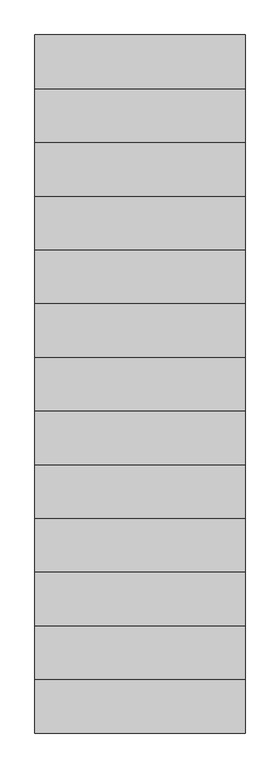
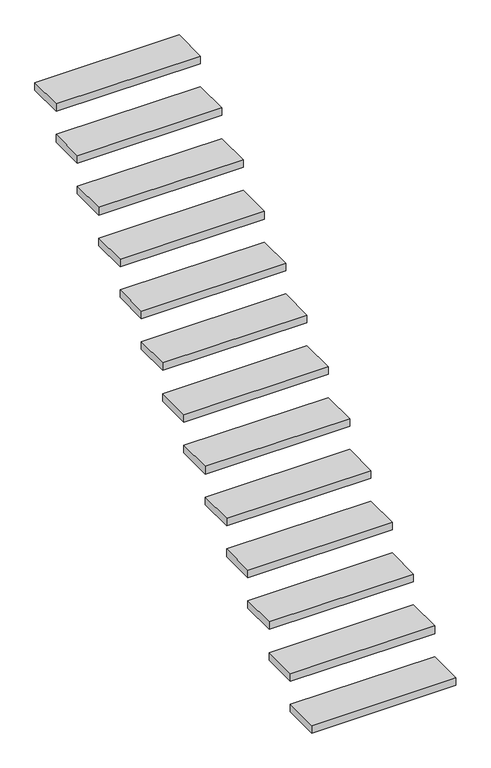
"""IFC4 building model written with IfcOpenShell, lengths in millimetres: stair geometry,   150414 :   150414."""

import ifcopenshell
import ifcopenshell.guid

model = None  # the IFC model being written
_history = None  # IfcOwnerHistory: only IFC2X3 demands one
_inside = {}  # id of a spatial element -> (the spatial element, [elements in it])
_under = {}  # id of a project, library or spatial element -> (it, [spatial elements below it])
_declared = {}  # id of a project -> (the project, [libraries it declares])
_typed = {}  # id of a type object -> (the type object, [elements of that type])
_made_of = {}  # id of a material, layer set ... -> (it, [elements and type objects made of it])


def new_model(schema):
    """Start an empty IFC model of exactly this schema.

    Asked for "IFC4X3", IfcOpenShell would pick the latest addendum, in which some entities
    have other attributes; the version numbers below select the first issue.
    IFC2X3 requires an IfcOwnerHistory on every rooted entity: one is made here for all.
    """
    global model, _history
    if schema == "IFC4X3":
        model = ifcopenshell.file(schema_version=(4, 3, 0, 0))
    else:
        model = ifcopenshell.file(schema=schema)
    _inside.clear()
    _under.clear()
    _declared.clear()
    _typed.clear()
    _made_of.clear()
    _history = None
    if model.schema == "IFC2X3":
        org = make("IfcOrganization", Name="unknown")
        user = make(
            "IfcPersonAndOrganization",
            ThePerson=make("IfcPerson", FamilyName="unknown"),
            TheOrganization=org,
        )
        app = make(
            "IfcApplication",
            ApplicationDeveloper=org,
            Version="unknown",
            ApplicationFullName="unknown",
            ApplicationIdentifier="unknown",
        )
        _history = make(
            "IfcOwnerHistory",
            OwningUser=user,
            OwningApplication=app,
            ChangeAction="ADDED",
            CreationDate=0,
        )
    return model


def make(cls, **values):
    """One entity of the class cls with the attributes given. An attribute that is None is left unset."""
    return model.create_entity(
        cls, **{name: value for name, value in values.items() if value is not None}
    )


def rooted(cls, **values):
    """An entity with a GlobalId (a new one), such as an element, a storey or a relation."""
    return make(cls, GlobalId=ifcopenshell.guid.new(), OwnerHistory=_history, **values)


def si_unit(unit_type, name, prefix=None):
    """IfcSIUnit, for example si_unit("LENGTHUNIT", "METRE", prefix="MILLI")."""
    return make("IfcSIUnit", UnitType=unit_type, Prefix=prefix, Name=name)


def assignment(units):
    """IfcUnitAssignment: the units of a project."""
    return None if units is None else make("IfcUnitAssignment", Units=units)


def point(xyz):
    """IfcCartesianPoint."""
    return None if xyz is None else make("IfcCartesianPoint", Coordinates=xyz)


def direction(xyz):
    """IfcDirection."""
    return None if xyz is None else make("IfcDirection", DirectionRatios=xyz)


def frame(location, z_axis=None, x_axis=None):
    """IfcAxis2Placement3D, a coordinate frame: its origin and axes. An axis left out is left unset."""
    return make(
        "IfcAxis2Placement3D",
        Location=point(location),
        Axis=direction(z_axis),
        RefDirection=direction(x_axis),
    )


def origin():
    """The frame at (0, 0, 0) with its axes left unset."""
    return frame((0.0, 0.0, 0.0))


def place(relative_to, where):
    """IfcLocalPlacement: puts the frame where relative to a parent placement (None: the world)."""
    return make(
        "IfcLocalPlacement", PlacementRelTo=relative_to, RelativePlacement=where
    )


def context(
    kind, dimensions, precision=None, world=None, true_north=None, identifier=None
):
    """IfcGeometricRepresentationContext, for example the 3D "Model" context."""
    return make(
        "IfcGeometricRepresentationContext",
        ContextIdentifier=identifier,
        ContextType=kind,
        CoordinateSpaceDimension=dimensions,
        Precision=precision,
        WorldCoordinateSystem=world,
        TrueNorth=true_north,
    )


def project(units=None, contexts=None):
    """IfcProject with its units and contexts."""
    return rooted(
        "IfcProject",
        Name="project",
        RepresentationContexts=contexts,
        UnitsInContext=assignment(units),
    )


def spatial(cls, under=None, at=None, **own):
    """A site, building, storey or space (cls), placed at a placement, below another one or the project."""
    s = rooted(cls, ObjectPlacement=at, **own)
    if under is not None:
        _under.setdefault(under.id(), (under, []))[1].append(s)
    return s


def polyline(points):
    """IfcPolyline through the points."""
    return make("IfcPolyline", Points=[point(p) for p in points])


def outline(outer, holes=None, kind="AREA"):
    """IfcArbitraryClosedProfileDef: a profile drawn as a closed curve; with holes, ...WithVoids."""
    if holes is None:
        return make("IfcArbitraryClosedProfileDef", ProfileType=kind, OuterCurve=outer)
    return make(
        "IfcArbitraryProfileDefWithVoids",
        ProfileType=kind,
        OuterCurve=outer,
        InnerCurves=holes,
    )


def extrude(swept, where, along, depth):
    """IfcExtrudedAreaSolid: the profile swept, set in the frame where, extruded along a direction by depth."""
    return make(
        "IfcExtrudedAreaSolid",
        SweptArea=swept,
        Position=where,
        ExtrudedDirection=direction(along),
        Depth=depth,
    )


def shape(context_of_items, identifier, shape_type, items):
    """IfcShapeRepresentation: the items that make up one representation, for example the "Body"."""
    return make(
        "IfcShapeRepresentation",
        ContextOfItems=context_of_items,
        RepresentationIdentifier=identifier,
        RepresentationType=shape_type,
        Items=items,
    )


def source(mapping_origin, context_of_items, identifier, shape_type, items):
    """IfcRepresentationMap: a shape defined once, which mapped items show again and again."""
    return make(
        "IfcRepresentationMap",
        MappingOrigin=mapping_origin,
        MappedRepresentation=shape(context_of_items, identifier, shape_type, items),
    )


def transform(
    local_origin,
    x_axis=None,
    y_axis=None,
    z_axis=None,
    scale=None,
    scale2=None,
    scale3=None,
    uniform=True,
):
    """IfcCartesianTransformationOperator3D, or its non-uniform kind. x_axis, y_axis, z_axis: its Axis1, 2, 3."""
    if uniform:
        return make(
            "IfcCartesianTransformationOperator3D",
            Axis1=direction(x_axis),
            Axis2=direction(y_axis),
            LocalOrigin=point(local_origin),
            Scale=scale,
            Axis3=direction(z_axis),
        )
    return make(
        "IfcCartesianTransformationOperator3DnonUniform",
        Axis1=direction(x_axis),
        Axis2=direction(y_axis),
        LocalOrigin=point(local_origin),
        Scale=scale,
        Axis3=direction(z_axis),
        Scale2=scale2,
        Scale3=scale3,
    )


def mapped(mapping_source, mapping_target):
    """IfcMappedItem: shows the shape of a source again, moved by a transform."""
    return make(
        "IfcMappedItem", MappingSource=mapping_source, MappingTarget=mapping_target
    )


def made_of(thing, what):
    """Note that an element or type object is made of a material, layer set ...; save() writes the relation."""
    if what is not None:
        _made_of.setdefault(what.id(), (what, []))[1].append(thing)
    return thing


def element(
    cls,
    number,
    at=None,
    inside=None,
    cuts=None,
    type_object=None,
    material=None,
    context=None,
    identifier="Body",
    shape_type=None,
    held_by="IfcProductDefinitionShape",
    body=None,
    shapes=None,
    **own,
):
    """One element of the class cls, such as IfcWall. Its Tag is "e" and its number.

    at: its placement. inside: the storey or other place that contains it. cuts: it is an
    opening in that element (IfcRelVoidsElement). A single representation is given by context,
    identifier, shape_type and body (its items); several are given by shapes. held_by: the class
    of the entity that holds the representations. save() writes the other relations.
    """
    e = rooted(cls, Tag="e%d" % number, ObjectPlacement=at, **own)
    if body is not None:
        shapes = [shape(context, identifier, shape_type, body)]
    if shapes is not None:
        e.Representation = make(held_by, Representations=shapes)
    if inside is not None:
        _inside.setdefault(inside.id(), (inside, []))[1].append(e)
    if cuts is not None:
        rooted(
            "IfcRelVoidsElement", RelatingBuildingElement=cuts, RelatedOpeningElement=e
        )
    if type_object is not None:
        _typed.setdefault(type_object.id(), (type_object, []))[1].append(e)
    return made_of(e, material)


def aggregate(whole, parts):
    """IfcRelAggregates: a whole, such as a stair, and the parts it consists of."""
    return rooted("IfcRelAggregates", RelatingObject=whole, RelatedObjects=parts)


def save(model, path):
    """Write the relations noted so far, then the file.

    IfcRelAggregates (storeys below a building ...), IfcRelContainedInSpatialStructure (elements
    in a storey), IfcRelDefinesByType, IfcRelAssociatesMaterial and IfcRelDeclares: one each for
    every whole, place, type object, material and project.
    """
    for whole, parts in _under.values():
        aggregate(whole, parts)
    for where, things in _inside.values():
        rooted(
            "IfcRelContainedInSpatialStructure",
            RelatedElements=things,
            RelatingStructure=where,
        )
    for kind, things in _typed.values():
        rooted("IfcRelDefinesByType", RelatedObjects=things, RelatingType=kind)
    for what, things in _made_of.values():
        rooted("IfcRelAssociatesMaterial", RelatedObjects=things, RelatingMaterial=what)
    for by, libraries in _declared.values():
        rooted("IfcRelDeclares", RelatingContext=by, RelatedDefinitions=libraries)
    model.write(path)


def stair_5d17669e(model_context):
    return source(origin(), model_context, "Body", "SweptSolid", [
        extrude(outline(polyline([(166797.7593015, 42144.7962965), (166797.7593015, 41914.7962965), (165897.7593015, 41914.7962965), (165897.7593015, 42144.7962965), (166797.7593015, 42144.7962965)])), frame((0.0, 0.0, 3482.1428571), z_axis=(0.0, 0.0, 1.0), x_axis=(1.0, 0.0, 0.0)), (0.0, 0.0, 1.0), 50.0),
        extrude(outline(polyline([(166797.7593015, 42374.7962965), (166797.7593015, 42144.7962965), (165897.7593015, 42144.7962965), (165897.7593015, 42374.7962965), (166797.7593015, 42374.7962965)])), frame((0.0, 0.0, 3684.2857143), z_axis=(0.0, 0.0, 1.0), x_axis=(1.0, 0.0, 0.0)), (0.0, 0.0, 1.0), 50.0),
        extrude(outline(polyline([(166797.7593015, 42604.7962965), (166797.7593015, 42374.7962965), (165897.7593015, 42374.7962965), (165897.7593015, 42604.7962965), (166797.7593015, 42604.7962965)])), frame((0.0, 0.0, 3886.4285714), z_axis=(0.0, 0.0, 1.0), x_axis=(1.0, 0.0, 0.0)), (0.0, 0.0, 1.0), 50.0),
        extrude(outline(polyline([(166797.7593015, 42834.7962965), (166797.7593015, 42604.7962965), (165897.7593015, 42604.7962965), (165897.7593015, 42834.7962965), (166797.7593015, 42834.7962965)])), frame((0.0, 0.0, 4088.5714286), z_axis=(0.0, 0.0, 1.0), x_axis=(1.0, 0.0, 0.0)), (0.0, 0.0, 1.0), 50.0),
        extrude(outline(polyline([(166797.7593015, 43064.7962965), (166797.7593015, 42834.7962965), (165897.7593015, 42834.7962965), (165897.7593015, 43064.7962965), (166797.7593015, 43064.7962965)])), frame((0.0, 0.0, 4290.7142857), z_axis=(0.0, 0.0, 1.0), x_axis=(1.0, 0.0, 0.0)), (0.0, 0.0, 1.0), 50.0),
        extrude(outline(polyline([(166797.7593015, 43294.7962965), (166797.7593015, 43064.7962965), (165897.7593015, 43064.7962965), (165897.7593015, 43294.7962965), (166797.7593015, 43294.7962965)])), frame((0.0, 0.0, 4492.8571429), z_axis=(0.0, 0.0, 1.0), x_axis=(1.0, 0.0, 0.0)), (0.0, 0.0, 1.0), 50.0),
        extrude(outline(polyline([(166797.7593015, 43524.7962965), (166797.7593015, 43294.7962965), (165897.7593015, 43294.7962965), (165897.7593015, 43524.7962965), (166797.7593015, 43524.7962965)])), frame((0.0, 0.0, 4695.0), z_axis=(0.0, 0.0, 1.0), x_axis=(1.0, 0.0, 0.0)), (0.0, 0.0, 1.0), 50.0),
        extrude(outline(polyline([(166797.7593015, 43754.7962965), (166797.7593015, 43524.7962965), (165897.7593015, 43524.7962965), (165897.7593015, 43754.7962965), (166797.7593015, 43754.7962965)])), frame((0.0, 0.0, 4897.1428571), z_axis=(0.0, 0.0, 1.0), x_axis=(1.0, 0.0, 0.0)), (0.0, 0.0, 1.0), 50.0),
        extrude(outline(polyline([(166797.7593015, 43984.7962965), (166797.7593015, 43754.7962965), (165897.7593015, 43754.7962965), (165897.7593015, 43984.7962965), (166797.7593015, 43984.7962965)])), frame((0.0, 0.0, 5099.2857143), z_axis=(0.0, 0.0, 1.0), x_axis=(1.0, 0.0, 0.0)), (0.0, 0.0, 1.0), 50.0),
        extrude(outline(polyline([(166797.7593015, 44214.7962965), (166797.7593015, 43984.7962965), (165897.7593015, 43984.7962965), (165897.7593015, 44214.7962965), (166797.7593015, 44214.7962965)])), frame((0.0, 0.0, 5301.4285714), z_axis=(0.0, 0.0, 1.0), x_axis=(1.0, 0.0, 0.0)), (0.0, 0.0, 1.0), 50.0),
        extrude(outline(polyline([(166797.7593015, 44444.7962965), (166797.7593015, 44214.7962965), (165897.7593015, 44214.7962965), (165897.7593015, 44444.7962965), (166797.7593015, 44444.7962965)])), frame((0.0, 0.0, 5503.5714286), z_axis=(0.0, 0.0, 1.0), x_axis=(1.0, 0.0, 0.0)), (0.0, 0.0, 1.0), 50.0),
        extrude(outline(polyline([(166797.7593015, 44674.7962965), (166797.7593015, 44444.7962965), (165897.7593015, 44444.7962965), (165897.7593015, 44674.7962965), (166797.7593015, 44674.7962965)])), frame((0.0, 0.0, 5705.7142857), z_axis=(0.0, 0.0, 1.0), x_axis=(1.0, 0.0, 0.0)), (0.0, 0.0, 1.0), 50.0),
        extrude(outline(polyline([(166797.7593015, 44904.7962965), (166797.7593015, 44674.7962965), (165897.7593015, 44674.7962965), (165897.7593015, 44904.7962965), (166797.7593015, 44904.7962965)])), frame((0.0, 0.0, 5907.8571429), z_axis=(0.0, 0.0, 1.0), x_axis=(1.0, 0.0, 0.0)), (0.0, 0.0, 1.0), 50.0),
    ])


if __name__ == "__main__":
    model = new_model("IFC4")
    model_context = context("Model", 3, world=origin())
    ifc_project = project(units=[si_unit("LENGTHUNIT", "METRE", prefix="MILLI")], contexts=[model_context])
    site = spatial("IfcSite", under=ifc_project)
    building = spatial("IfcBuilding", under=site)
    placement = place(None, origin())
    stair_shape = stair_5d17669e(model_context)
    element("IfcStair", 1, ObjectType="  150414 :   150414", at=placement, inside=building, context=model_context, shape_type="MappedRepresentation", body=[
        mapped(stair_shape, transform((0.0, 0.0, 0.0), x_axis=(1.0, 0.0, 0.0), y_axis=(0.0, 1.0, 0.0), z_axis=(0.0, 0.0, 1.0))),
    ])
    save(model, "model.ifc")

# Revit data of these elements
# Type "  150414 :   150414"
#   Abrechnungsart = "St"
#   Allright_Bauteil_ID = "0131Tre0659044575"
#   Codetext = "TR-MASSIV-GER\\"
#   Material = "Stahlbeton"
#   Objektname = "Treppe"
#   NameOverride = " "
#   Reference = "STB-Treppe"
#   ThermalTransmittance = 0.0000 BTU/(h·ft²·°F)
#   NosingLength = 0.000 m
#   NumberOfRiser = 14
#   NumberOfTreads = 13
#   RiserHeight = 2.021 m
#   TreadLength = 2.300 m
#   IsExternal = no
#   FireExit = no
#   HandicapAccessible = no
#   HasNonSkidSurface = no
# Element 1 (IfcStair, "  150414 :   150414")
#   Materials on its faces: "weiss"
# Materials
#   "weiss": class "Unassigned", colour RGB 255 255 255, transparency 0
